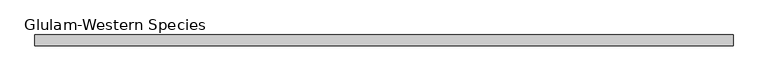
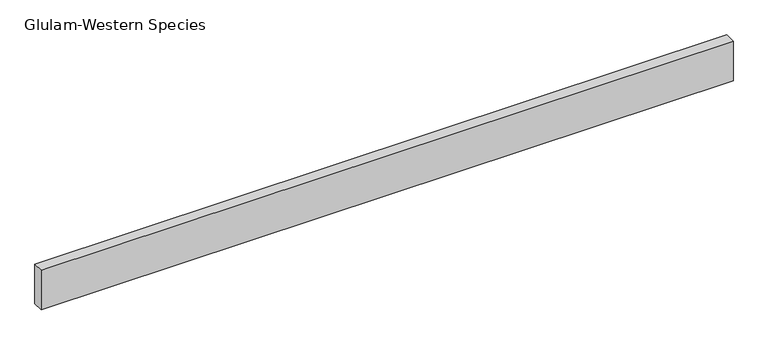
"""IFC4 building model written with IfcOpenShell, lengths in millimetres: beam geometry, Glulam-Western Species : 3.125x12 Headers Exterior."""

from ifc_helpers import new_model, si_unit, frame, origin, place, context, project, spatial, polyline, outline, extrude, source, transform, mapped, element, save


def glulam_western_species_20871a06(model_context):
    return source(origin(), model_context, "Body", "SweptSolid", [
        extrude(outline(polyline([(481.409375, 39.6875), (481.409375, -39.6875), (-4547.790625, -39.6875), (-4547.790625, 39.6875), (481.409375, 39.6875)])), frame((0.0, 0.0, -152.4), z_axis=(0.0, 0.0, 1.0), x_axis=(1.0, 0.0, 0.0)), (0.0, 0.0, 1.0), 304.8),
    ])


if __name__ == "__main__":
    model = new_model("IFC4")
    model_context = context("Model", 3, world=origin())
    ifc_project = project(units=[si_unit("LENGTHUNIT", "METRE", prefix="MILLI")], contexts=[model_context])
    site = spatial("IfcSite", under=ifc_project)
    building = spatial("IfcBuilding", under=site)
    placement = place(None, origin())
    glulam_western_species_shape = glulam_western_species_20871a06(model_context)
    element("IfcBeam", 1, ObjectType="Glulam-Western Species : 3.125x12 Headers Exterior", at=placement, inside=building, context=model_context, shape_type="MappedRepresentation", body=[
        mapped(glulam_western_species_shape, transform((0.0, 0.0, 0.0), x_axis=(1.0, 0.0, 0.0), y_axis=(0.0, 1.0, 0.0), z_axis=(0.0, 0.0, 1.0))),
    ])
    save(model, "model.ifc")

# Revit data of these elements
# Type "Glulam-Western Species : 3.125x12 Headers Exterior"
#   Assembly Code = "B10"
#   Laminations = "8"
#   A = 0.260417 SF
#   Ix = 450
#   Iy = 30.52
#   Length [instance default] = 5' - 0"
#   Sx = 75
#   Sy = 19.53
#   b = 0' - 3 1/8"
#   d = 1' - 0"
#   Structural Material [instance default] = Softwood, Lumber
# Element 1 (IfcBeam, "Glulam-Western Species : 3.125x12 Headers Exterior")
#   Structural Material = Douglas Fir #2
#   Materials on its faces: "Douglas Fir #2"
# Materials
#   "Softwood, Lumber": class "Wood", colour RGB 223 192 134, transparency 0, Description = "Pinus Echinata", Cost = 0
#   "Douglas Fir #2": class "Wood", colour RGB 223 192 134, transparency 0, Description = "Pinus Echinata", Cost = 0
